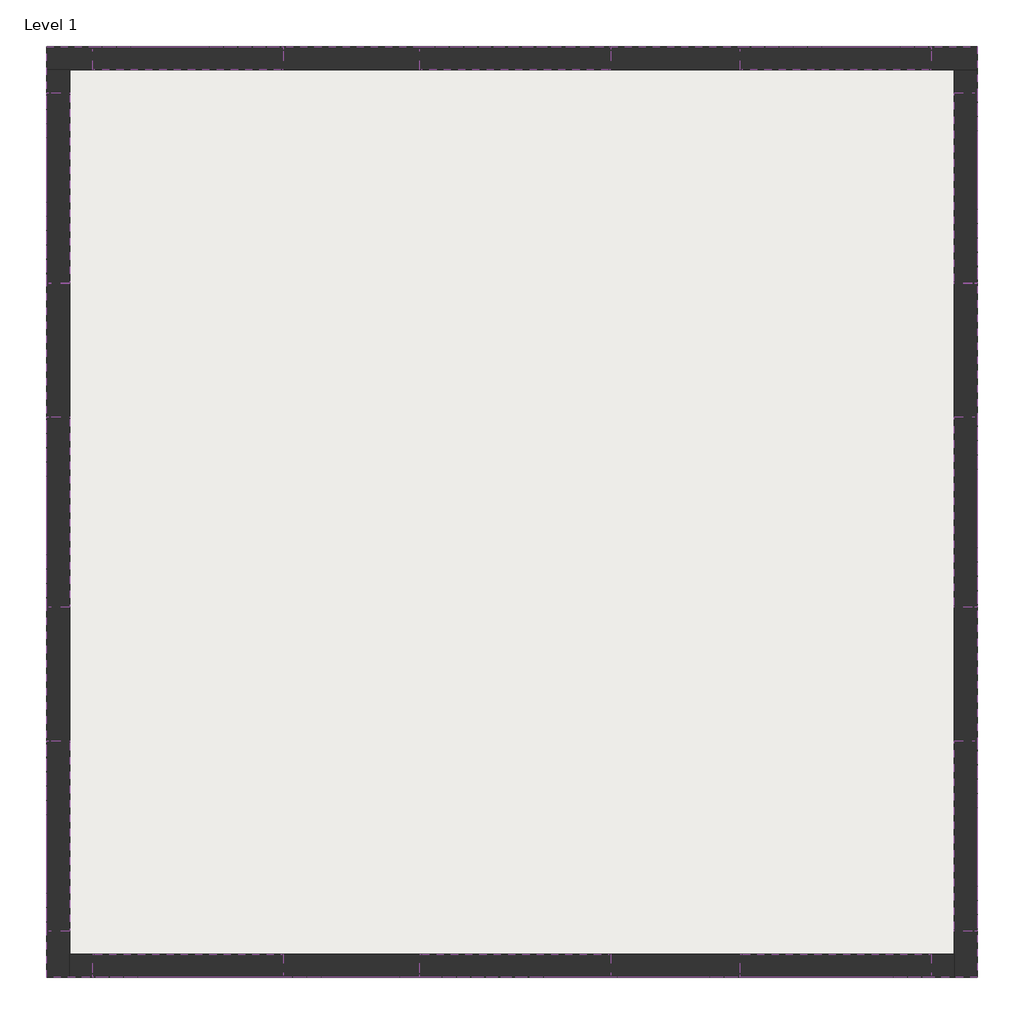
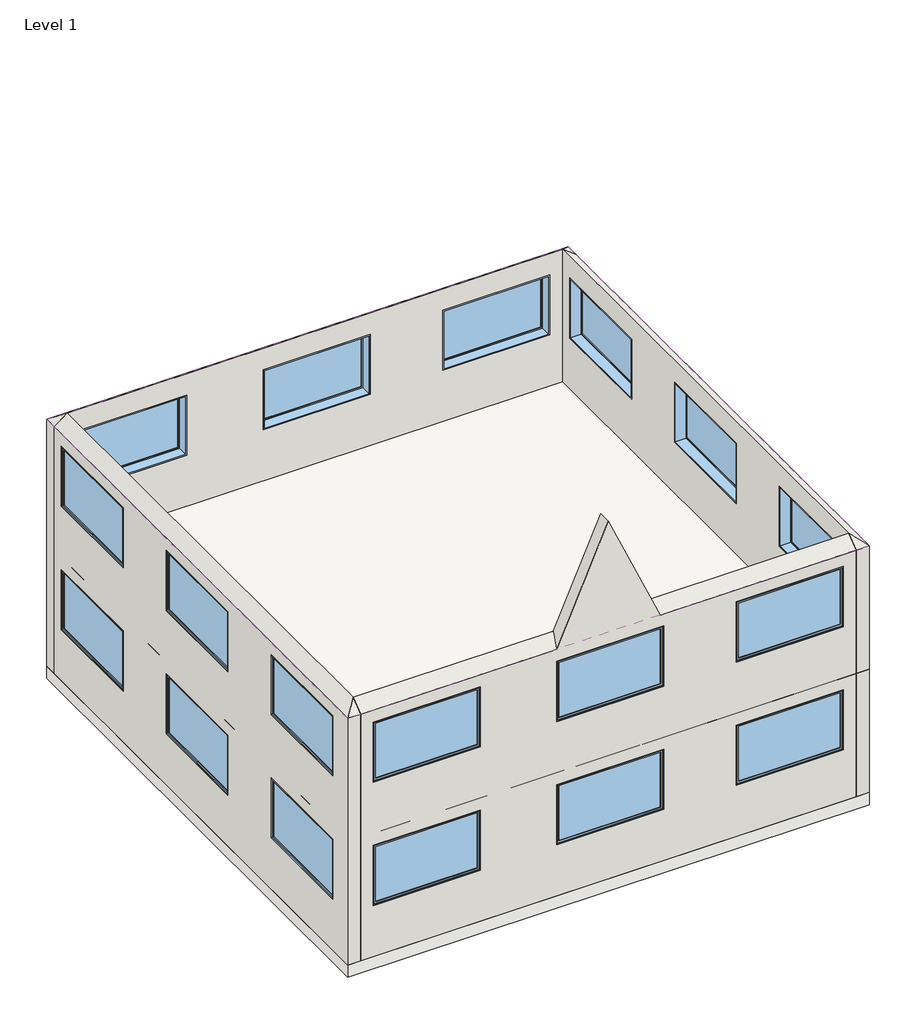
# One storey: 24 windows, 4 walls, 2 slabs, 1 roof.
"""IFC4 building model written with IfcOpenShell, lengths in millimetres."""

import ifcopenshell
import ifcopenshell.guid

model = None  # the IFC model being written
_history = None  # IfcOwnerHistory: only IFC2X3 demands one
_inside = {}  # id of a spatial element -> (the spatial element, [elements in it])
_under = {}  # id of a project, library or spatial element -> (it, [spatial elements below it])
_declared = {}  # id of a project -> (the project, [libraries it declares])
_typed = {}  # id of a type object -> (the type object, [elements of that type])
_made_of = {}  # id of a material, layer set ... -> (it, [elements and type objects made of it])


def new_model(schema):
    """Start an empty IFC model of exactly this schema.

    Asked for "IFC4X3", IfcOpenShell would pick the latest addendum, in which some entities
    have other attributes; the version numbers below select the first issue.
    IFC2X3 requires an IfcOwnerHistory on every rooted entity: one is made here for all.
    """
    global model, _history
    if schema == "IFC4X3":
        model = ifcopenshell.file(schema_version=(4, 3, 0, 0))
    else:
        model = ifcopenshell.file(schema=schema)
    _inside.clear()
    _under.clear()
    _declared.clear()
    _typed.clear()
    _made_of.clear()
    _history = None
    if model.schema == "IFC2X3":
        org = make("IfcOrganization", Name="unknown")
        user = make(
            "IfcPersonAndOrganization",
            ThePerson=make("IfcPerson", FamilyName="unknown"),
            TheOrganization=org,
        )
        app = make(
            "IfcApplication",
            ApplicationDeveloper=org,
            Version="unknown",
            ApplicationFullName="unknown",
            ApplicationIdentifier="unknown",
        )
        _history = make(
            "IfcOwnerHistory",
            OwningUser=user,
            OwningApplication=app,
            ChangeAction="ADDED",
            CreationDate=0,
        )
    return model


def make(cls, **values):
    """One entity of the class cls with the attributes given. An attribute that is None is left unset."""
    return model.create_entity(
        cls, **{name: value for name, value in values.items() if value is not None}
    )


def rooted(cls, **values):
    """An entity with a GlobalId (a new one), such as an element, a storey or a relation."""
    return make(cls, GlobalId=ifcopenshell.guid.new(), OwnerHistory=_history, **values)


def si_unit(unit_type, name, prefix=None):
    """IfcSIUnit, for example si_unit("LENGTHUNIT", "METRE", prefix="MILLI")."""
    return make("IfcSIUnit", UnitType=unit_type, Prefix=prefix, Name=name)


def assignment(units):
    """IfcUnitAssignment: the units of a project."""
    return None if units is None else make("IfcUnitAssignment", Units=units)


def point(xyz):
    """IfcCartesianPoint."""
    return None if xyz is None else make("IfcCartesianPoint", Coordinates=xyz)


def direction(xyz):
    """IfcDirection."""
    return None if xyz is None else make("IfcDirection", DirectionRatios=xyz)


def frame(location, z_axis=None, x_axis=None):
    """IfcAxis2Placement3D, a coordinate frame: its origin and axes. An axis left out is left unset."""
    return make(
        "IfcAxis2Placement3D",
        Location=point(location),
        Axis=direction(z_axis),
        RefDirection=direction(x_axis),
    )


def origin():
    """The frame at (0, 0, 0) with its axes left unset."""
    return frame((0.0, 0.0, 0.0))


def place(relative_to, where):
    """IfcLocalPlacement: puts the frame where relative to a parent placement (None: the world)."""
    return make(
        "IfcLocalPlacement", PlacementRelTo=relative_to, RelativePlacement=where
    )


def context(
    kind, dimensions, precision=None, world=None, true_north=None, identifier=None
):
    """IfcGeometricRepresentationContext, for example the 3D "Model" context."""
    return make(
        "IfcGeometricRepresentationContext",
        ContextIdentifier=identifier,
        ContextType=kind,
        CoordinateSpaceDimension=dimensions,
        Precision=precision,
        WorldCoordinateSystem=world,
        TrueNorth=true_north,
    )


def project(units=None, contexts=None):
    """IfcProject with its units and contexts."""
    return rooted(
        "IfcProject",
        Name="project",
        RepresentationContexts=contexts,
        UnitsInContext=assignment(units),
    )


def spatial(cls, under=None, at=None, **own):
    """A site, building, storey or space (cls), placed at a placement, below another one or the project."""
    s = rooted(cls, ObjectPlacement=at, **own)
    if under is not None:
        _under.setdefault(under.id(), (under, []))[1].append(s)
    return s


def polyline(points):
    """IfcPolyline through the points."""
    return make("IfcPolyline", Points=[point(p) for p in points])


def outline(outer, holes=None, kind="AREA"):
    """IfcArbitraryClosedProfileDef: a profile drawn as a closed curve; with holes, ...WithVoids."""
    if holes is None:
        return make("IfcArbitraryClosedProfileDef", ProfileType=kind, OuterCurve=outer)
    return make(
        "IfcArbitraryProfileDefWithVoids",
        ProfileType=kind,
        OuterCurve=outer,
        InnerCurves=holes,
    )


def extrude(swept, where, along, depth):
    """IfcExtrudedAreaSolid: the profile swept, set in the frame where, extruded along a direction by depth."""
    return make(
        "IfcExtrudedAreaSolid",
        SweptArea=swept,
        Position=where,
        ExtrudedDirection=direction(along),
        Depth=depth,
    )


def faces_of(points, faces, orient=None, outer=None):
    """IfcFace entities. A face is a list of loops; a loop is a list of indices into points, from 0.

    orient and outer hold one flag for each loop. By default every Orientation is true, the
    first loop of a face is its IfcFaceOuterBound and the others are IfcFaceBound.
    """
    made = []
    for i, loops in enumerate(faces):
        bounds = []
        for j, loop in enumerate(loops):
            is_outer = j == 0 if outer is None else outer[i][j]
            bounds.append(
                make(
                    "IfcFaceOuterBound" if is_outer else "IfcFaceBound",
                    Bound=make("IfcPolyLoop", Polygon=[points[k] for k in loop]),
                    Orientation=True if orient is None else orient[i][j],
                )
            )
        made.append(make("IfcFace", Bounds=bounds))
    return made


def faceted_brep(points, faces, orient=None, outer=None, voids=None):
    """IfcFacetedBrep: a solid bounded by flat faces; with voids (closed shells), ...WithVoids."""
    shared = [point(p) for p in points]
    hull = make("IfcClosedShell", CfsFaces=faces_of(shared, faces, orient, outer))
    if voids is None:
        return make("IfcFacetedBrep", Outer=hull)
    return make(
        "IfcFacetedBrepWithVoids",
        Outer=hull,
        Voids=[
            make(cls, CfsFaces=faces_of(shared, fs, o, b)) for cls, fs, o, b in voids
        ],
    )


def shape(context_of_items, identifier, shape_type, items):
    """IfcShapeRepresentation: the items that make up one representation, for example the "Body"."""
    return make(
        "IfcShapeRepresentation",
        ContextOfItems=context_of_items,
        RepresentationIdentifier=identifier,
        RepresentationType=shape_type,
        Items=items,
    )


def source(mapping_origin, context_of_items, identifier, shape_type, items):
    """IfcRepresentationMap: a shape defined once, which mapped items show again and again."""
    return make(
        "IfcRepresentationMap",
        MappingOrigin=mapping_origin,
        MappedRepresentation=shape(context_of_items, identifier, shape_type, items),
    )


def transform(
    local_origin,
    x_axis=None,
    y_axis=None,
    z_axis=None,
    scale=None,
    scale2=None,
    scale3=None,
    uniform=True,
):
    """IfcCartesianTransformationOperator3D, or its non-uniform kind. x_axis, y_axis, z_axis: its Axis1, 2, 3."""
    if uniform:
        return make(
            "IfcCartesianTransformationOperator3D",
            Axis1=direction(x_axis),
            Axis2=direction(y_axis),
            LocalOrigin=point(local_origin),
            Scale=scale,
            Axis3=direction(z_axis),
        )
    return make(
        "IfcCartesianTransformationOperator3DnonUniform",
        Axis1=direction(x_axis),
        Axis2=direction(y_axis),
        LocalOrigin=point(local_origin),
        Scale=scale,
        Axis3=direction(z_axis),
        Scale2=scale2,
        Scale3=scale3,
    )


def mapped(mapping_source, mapping_target):
    """IfcMappedItem: shows the shape of a source again, moved by a transform."""
    return make(
        "IfcMappedItem", MappingSource=mapping_source, MappingTarget=mapping_target
    )


def made_of(thing, what):
    """Note that an element or type object is made of a material, layer set ...; save() writes the relation."""
    if what is not None:
        _made_of.setdefault(what.id(), (what, []))[1].append(thing)
    return thing


def element(
    cls,
    number,
    at=None,
    inside=None,
    cuts=None,
    type_object=None,
    material=None,
    context=None,
    identifier="Body",
    shape_type=None,
    held_by="IfcProductDefinitionShape",
    body=None,
    shapes=None,
    **own,
):
    """One element of the class cls, such as IfcWall. Its Tag is "e" and its number.

    at: its placement. inside: the storey or other place that contains it. cuts: it is an
    opening in that element (IfcRelVoidsElement). A single representation is given by context,
    identifier, shape_type and body (its items); several are given by shapes. held_by: the class
    of the entity that holds the representations. save() writes the other relations.
    """
    e = rooted(cls, Tag="e%d" % number, ObjectPlacement=at, **own)
    if body is not None:
        shapes = [shape(context, identifier, shape_type, body)]
    if shapes is not None:
        e.Representation = make(held_by, Representations=shapes)
    if inside is not None:
        _inside.setdefault(inside.id(), (inside, []))[1].append(e)
    if cuts is not None:
        rooted(
            "IfcRelVoidsElement", RelatingBuildingElement=cuts, RelatedOpeningElement=e
        )
    if type_object is not None:
        _typed.setdefault(type_object.id(), (type_object, []))[1].append(e)
    return made_of(e, material)


def aggregate(whole, parts):
    """IfcRelAggregates: a whole, such as a stair, and the parts it consists of."""
    return rooted("IfcRelAggregates", RelatingObject=whole, RelatedObjects=parts)


def save(model, path):
    """Write the relations noted so far, then the file.

    IfcRelAggregates (storeys below a building ...), IfcRelContainedInSpatialStructure (elements
    in a storey), IfcRelDefinesByType, IfcRelAssociatesMaterial and IfcRelDeclares: one each for
    every whole, place, type object, material and project.
    """
    for whole, parts in _under.values():
        aggregate(whole, parts)
    for where, things in _inside.values():
        rooted(
            "IfcRelContainedInSpatialStructure",
            RelatedElements=things,
            RelatingStructure=where,
        )
    for kind, things in _typed.values():
        rooted("IfcRelDefinesByType", RelatedObjects=things, RelatingType=kind)
    for what, things in _made_of.values():
        rooted("IfcRelAssociatesMaterial", RelatedObjects=things, RelatingMaterial=what)
    for by, libraries in _declared.values():
        rooted("IfcRelDeclares", RelatingContext=by, RelatedDefinitions=libraries)
    model.write(path)


def m_fixed_2500_x_1486mm_baf7df51(model_context):
    return source(origin(), model_context, "Body", "SweptSolid", [
        extrude(outline(polyline([(-1187.0, 130.4), (1187.0, 130.4), (1187.0, 118.4), (-1187.0, 118.4), (-1187.0, 130.4)])), frame((0.0, 0.0, 978.0), z_axis=(0.0, 0.0, 1.0), x_axis=(1.0, 0.0, 0.0)), (0.0, 0.0, 1.0), 1360.5),
        extrude(outline(polyline([(2382.5, -1231.0), (934.0, -1231.0), (934.0, 1231.0), (2382.5, 1231.0), (2382.5, -1231.0)]), holes=[polyline([(2338.5, -1187.0), (2338.5, 1187.0), (978.0, 1187.0), (978.0, -1187.0), (2338.5, -1187.0)])]), frame((0.0, 102.4, 0.0), z_axis=(0.0, 1.0, 0.0), x_axis=(0.0, 0.0, 1.0)), (0.0, 0.0, 1.0), 44.0),
        extrude(outline(polyline([(2401.5, -1250.0), (915.0, -1250.0), (915.0, 1250.0), (2401.5, 1250.0), (2401.5, -1250.0)]), holes=[polyline([(2382.5, -1231.0), (2382.5, 1231.0), (934.0, 1231.0), (934.0, -1231.0), (2382.5, -1231.0)])]), frame((0.0, 102.4, 0.0), z_axis=(0.0, 1.0, 0.0), x_axis=(0.0, 0.0, 1.0)), (0.0, 0.0, 1.0), 63.0),
        extrude(outline(polyline([(2401.5, -1250.0), (915.0, -1250.0), (915.0, 1250.0), (2401.5, 1250.0), (2401.5, -1250.0)]), holes=[polyline([(2369.5, -1218.0), (2369.5, 1218.0), (947.0, 1218.0), (947.0, -1218.0), (2369.5, -1218.0)])]), frame((0.0, -139.4, 0.0), z_axis=(0.0, 1.0, 0.0), x_axis=(0.0, 0.0, 1.0)), (0.0, 0.0, 1.0), 241.8),
    ])


def m_fixed_2500_x_1486mm_49bc14c1(model_context):
    return source(origin(), model_context, "Body", "SweptSolid", [
        extrude(outline(polyline([(-1187.0, -130.4), (-1187.0, -118.4), (1187.0, -118.4), (1187.0, -130.4), (-1187.0, -130.4)])), frame((0.0, 0.0, 978.0), z_axis=(0.0, 0.0, 1.0), x_axis=(1.0, 0.0, 0.0)), (0.0, 0.0, 1.0), 1360.5),
        extrude(outline(polyline([(2382.5, -1231.0), (934.0, -1231.0), (934.0, 1231.0), (2382.5, 1231.0), (2382.5, -1231.0)]), holes=[polyline([(2338.5, -1187.0), (2338.5, 1187.0), (978.0, 1187.0), (978.0, -1187.0), (2338.5, -1187.0)])]), frame((0.0, -146.4, 0.0), z_axis=(0.0, 1.0, 0.0), x_axis=(0.0, 0.0, 1.0)), (0.0, 0.0, 1.0), 44.0),
        extrude(outline(polyline([(2401.5, -1250.0), (915.0, -1250.0), (915.0, 1250.0), (2401.5, 1250.0), (2401.5, -1250.0)]), holes=[polyline([(2382.5, -1231.0), (2382.5, 1231.0), (934.0, 1231.0), (934.0, -1231.0), (2382.5, -1231.0)])]), frame((0.0, -165.4, 0.0), z_axis=(0.0, 1.0, 0.0), x_axis=(0.0, 0.0, 1.0)), (0.0, 0.0, 1.0), 63.0),
        extrude(outline(polyline([(2401.5, -1250.0), (915.0, -1250.0), (915.0, 1250.0), (2401.5, 1250.0), (2401.5, -1250.0)]), holes=[polyline([(2369.5, -1218.0), (2369.5, 1218.0), (947.0, 1218.0), (947.0, -1218.0), (2369.5, -1218.0)])]), frame((0.0, -102.4, 0.0), z_axis=(0.0, 1.0, 0.0), x_axis=(0.0, 0.0, 1.0)), (0.0, 0.0, 1.0), 241.8),
    ])


model = new_model("IFC4")

# Units and contexts
model_context = context("Model", 3, world=origin())
ifc_project = project(units=[si_unit("LENGTHUNIT", "METRE", prefix="MILLI")], contexts=[model_context])

# Site, building, storey
site = spatial("IfcSite", under=ifc_project)
building = spatial("IfcBuilding", under=site)
storey = spatial("IfcBuildingStorey", under=building, Name="Level 1", Elevation=0.0)

# Roof
placement = place(None, origin())
element("IfcRoof", 1, ObjectType="Generic Roof - 300mm", at=placement, inside=storey, context=model_context, shape_type="Brep", body=[
    faceted_brep([(21465.644102, 9062.7173115, 6096.0), (15369.644102, 2966.7173115, 10668.0170156), (9273.644102, 9062.7173115, 6096.0), (9273.644102, -3129.2826885, 6096.0), (14160.6176554, -3129.2826885, 6096.0), (13998.044102, -3129.2826885, 6096.0), (21465.644102, -3129.2826885, 6096.0), (16741.244102, -3129.2826885, 6096.0), (16578.6705485, -3129.2826885, 6096.0), (15369.644102, 528.4582497, 8839.3159134), (15369.644102, -3129.2826885, 8839.3159134), (21465.644102, 9062.7173115, 6471.0005024), (9273.644102, 9062.7173115, 6471.0005024), (15369.644102, 2966.7173115, 11043.0175181), (9273.644102, -3129.2826885, 6471.0005024), (13998.044102, -3129.2826885, 6471.0005024), (15369.644102, 1020.3018679, 9583.2005024), (16741.244102, -3129.2826885, 6471.0005024), (21465.644102, -3129.2826885, 6471.0005024), (15369.644102, -3129.2826885, 9583.2005024)], [[[0, 1, 2]], [[2, 1, 3]], [[4, 5, 3, 1, 6, 7, 8, 9]], [[6, 1, 0]], [[4, 9, 10]], [[8, 10, 9]], [[11, 12, 13]], [[12, 14, 13]], [[15, 16, 17, 18, 13, 14]], [[18, 11, 13]], [[15, 19, 16]], [[17, 16, 19]], [[6, 18, 17, 7]], [[0, 11, 18, 6]], [[2, 12, 11, 0]], [[3, 14, 12, 2]], [[5, 15, 14, 3]], [[17, 19, 15, 5, 4, 10, 8, 7]]]),
])

# Slabs
element("IfcSlab", 2, ObjectType="Generic Floor - 304.8mm", at=placement, inside=storey, context=model_context, shape_type="Brep", body=[
    faceted_brep([(21465.644102, 9062.7173115, -304.8), (21465.644102, -3129.2826885, -304.8), (9273.644102, -3129.2826885, -304.8), (9273.644102, 9062.7173115, -304.8), (21465.644102, 9062.7173115, 0.0), (9273.644102, 9062.7173115, 0.0), (9273.644102, -3129.2826885, 0.0), (9578.444102, -3129.2826885, 0.0), (21160.844102, -3129.2826885, 0.0), (21465.644102, -3129.2826885, 0.0), (21465.644102, 8757.9173115, 0.0)], [[[0, 1, 2, 3]], [[4, 5, 6, 7, 8, 9, 10]], [[1, 0, 4, 10, 9]], [[2, 1, 9, 8, 7, 6]], [[3, 2, 6, 5]], [[0, 3, 5, 4]]]),
])
element("IfcSlab", 3, ObjectType="Generic Floor - 304.8mm", at=placement, inside=storey, context=model_context, shape_type="SweptSolid", body=[
    extrude(outline(polyline([(21465.644102, 9062.7173115), (21465.644102, -3129.2826885), (9273.644102, -3129.2826885), (9273.644102, 9062.7173115), (21465.644102, 9062.7173115)])), frame((0.0, 0.0, 2743.2), z_axis=(0.0, 0.0, 1.0), x_axis=(1.0, 0.0, 0.0)), (0.0, 0.0, 1.0), 304.8),
])

# Walls
element("IfcWall", 4, ObjectType="Generic - 304.8mm", at=placement, inside=storey, context=model_context, shape_type="Brep", body=[
    faceted_brep([(9273.644102, 8757.9173115, 0.0), (9578.444102, 8757.9173115, 0.0), (21160.844102, 8757.9173115, 0.0), (21465.644102, 8757.9173115, 0.0), (21465.644102, 8757.9173115, 6096.0), (21160.844102, 8757.9173115, 6324.6008508), (9578.444102, 8757.9173115, 6324.6008508), (9273.644102, 8757.9173115, 6096.0), (14163.244102, 8757.9173115, 4309.5), (14163.244102, 8757.9173115, 5796.0), (16663.244102, 8757.9173115, 5796.0), (16663.244102, 8757.9173115, 4309.5), (9876.044102, 8757.9173115, 4309.5), (9876.044102, 8757.9173115, 5796.0), (12376.044102, 8757.9173115, 5796.0), (12376.044102, 8757.9173115, 4309.5), (18363.244102, 8757.9173115, 4309.5), (18363.244102, 8757.9173115, 5796.0), (20863.244102, 8757.9173115, 5796.0), (20863.244102, 8757.9173115, 4309.5), (18363.244102, 8757.9173115, 1261.5), (18363.244102, 8757.9173115, 2748.0), (20863.244102, 8757.9173115, 2748.0), (20863.244102, 8757.9173115, 1261.5), (9876.044102, 8757.9173115, 1261.5), (9876.044102, 8757.9173115, 2748.0), (12376.044102, 8757.9173115, 2748.0), (12376.044102, 8757.9173115, 1261.5), (14163.244102, 8757.9173115, 1261.5), (14163.244102, 8757.9173115, 2748.0), (16663.244102, 8757.9173115, 2748.0), (16663.244102, 8757.9173115, 1261.5), (9273.644102, 9062.7173115, 0.0), (9273.644102, 9062.7173115, 6096.0), (21465.644102, 9062.7173115, 6096.0), (21465.644102, 9062.7173115, 0.0), (14163.244102, 9062.7173115, 4309.5), (16663.244102, 9062.7173115, 4309.5), (16663.244102, 9062.7173115, 5796.0), (14163.244102, 9062.7173115, 5796.0), (9876.044102, 9062.7173115, 4309.5), (12376.044102, 9062.7173115, 4309.5), (12376.044102, 9062.7173115, 5796.0), (9876.044102, 9062.7173115, 5796.0), (18363.244102, 9062.7173115, 4309.5), (20863.244102, 9062.7173115, 4309.5), (20863.244102, 9062.7173115, 5796.0), (18363.244102, 9062.7173115, 5796.0), (18363.244102, 9062.7173115, 1261.5), (20863.244102, 9062.7173115, 1261.5), (20863.244102, 9062.7173115, 2748.0), (18363.244102, 9062.7173115, 2748.0), (9876.044102, 9062.7173115, 1261.5), (12376.044102, 9062.7173115, 1261.5), (12376.044102, 9062.7173115, 2748.0), (9876.044102, 9062.7173115, 2748.0), (14163.244102, 9062.7173115, 1261.5), (16663.244102, 9062.7173115, 1261.5), (16663.244102, 9062.7173115, 2748.0), (14163.244102, 9062.7173115, 2748.0)], [[[0, 1, 2, 3, 4, 5, 6, 7], [8, 9, 10, 11], [12, 13, 14, 15], [16, 17, 18, 19], [20, 21, 22, 23], [24, 25, 26, 27], [28, 29, 30, 31]], [[32, 33, 34, 35], [36, 37, 38, 39], [40, 41, 42, 43], [44, 45, 46, 47], [48, 49, 50, 51], [52, 53, 54, 55], [56, 57, 58, 59]], [[3, 2, 1, 0, 32, 35]], [[4, 3, 35, 34]], [[0, 7, 33, 32]], [[9, 8, 36, 39]], [[10, 9, 39, 38]], [[11, 10, 38, 37]], [[8, 11, 37, 36]], [[13, 12, 40, 43]], [[14, 13, 43, 42]], [[15, 14, 42, 41]], [[12, 15, 41, 40]], [[17, 16, 44, 47]], [[18, 17, 47, 46]], [[19, 18, 46, 45]], [[16, 19, 45, 44]], [[21, 20, 48, 51]], [[22, 21, 51, 50]], [[23, 22, 50, 49]], [[20, 23, 49, 48]], [[25, 24, 52, 55]], [[26, 25, 55, 54]], [[27, 26, 54, 53]], [[24, 27, 53, 52]], [[29, 28, 56, 59]], [[30, 29, 59, 58]], [[31, 30, 58, 57]], [[28, 31, 57, 56]], [[7, 6, 33]], [[6, 5, 34, 33]], [[5, 4, 34]]]),
])
element("IfcWall", 5, ObjectType="Generic - 304.8mm", at=placement, inside=storey, context=model_context, shape_type="Brep", body=[
    faceted_brep([(21160.844102, 8757.9173115, 0.0), (21160.844102, -2824.4826885, 0.0), (21160.844102, -3129.2826885, 0.0), (21160.844102, -3129.2826885, 6096.0), (21160.844102, -2824.4826885, 6324.6008508), (21160.844102, 8757.9173115, 6324.6008508), (21160.844102, -26.8826885, 4309.5), (21160.844102, -26.8826885, 5796.0), (21160.844102, -2526.8826885, 5796.0), (21160.844102, -2526.8826885, 4309.5), (21160.844102, 8460.3173115, 4309.5), (21160.844102, 8460.3173115, 5796.0), (21160.844102, 5960.3173115, 5796.0), (21160.844102, 5960.3173115, 4309.5), (21160.844102, 4216.7173115, 4309.5), (21160.844102, 4216.7173115, 5796.0), (21160.844102, 1716.7173115, 5796.0), (21160.844102, 1716.7173115, 4309.5), (21160.844102, 4216.7173115, 1261.5), (21160.844102, 4216.7173115, 2748.0), (21160.844102, 1716.7173115, 2748.0), (21160.844102, 1716.7173115, 1261.5), (21160.844102, 8460.3173115, 1261.5), (21160.844102, 8460.3173115, 2748.0), (21160.844102, 5960.3173115, 2748.0), (21160.844102, 5960.3173115, 1261.5), (21160.844102, -26.8826885, 1261.5), (21160.844102, -26.8826885, 2748.0), (21160.844102, -2526.8826885, 2748.0), (21160.844102, -2526.8826885, 1261.5), (21465.644102, 8757.9173115, 0.0), (21465.644102, 8757.9173115, 6096.0), (21465.644102, -3129.2826885, 6096.0), (21465.644102, -3129.2826885, 0.0), (21465.644102, -26.8826885, 4309.5), (21465.644102, -2526.8826885, 4309.5), (21465.644102, -2526.8826885, 5796.0), (21465.644102, -26.8826885, 5796.0), (21465.644102, 8460.3173115, 4309.5), (21465.644102, 5960.3173115, 4309.5), (21465.644102, 5960.3173115, 5796.0), (21465.644102, 8460.3173115, 5796.0), (21465.644102, 4216.7173115, 4309.5), (21465.644102, 1716.7173115, 4309.5), (21465.644102, 1716.7173115, 5796.0), (21465.644102, 4216.7173115, 5796.0), (21465.644102, 4216.7173115, 1261.5), (21465.644102, 1716.7173115, 1261.5), (21465.644102, 1716.7173115, 2748.0), (21465.644102, 4216.7173115, 2748.0), (21465.644102, 8460.3173115, 1261.5), (21465.644102, 5960.3173115, 1261.5), (21465.644102, 5960.3173115, 2748.0), (21465.644102, 8460.3173115, 2748.0), (21465.644102, -26.8826885, 1261.5), (21465.644102, -2526.8826885, 1261.5), (21465.644102, -2526.8826885, 2748.0), (21465.644102, -26.8826885, 2748.0)], [[[0, 1, 2, 3, 4, 5], [6, 7, 8, 9], [10, 11, 12, 13], [14, 15, 16, 17], [18, 19, 20, 21], [22, 23, 24, 25], [26, 27, 28, 29]], [[30, 31, 32, 33], [34, 35, 36, 37], [38, 39, 40, 41], [42, 43, 44, 45], [46, 47, 48, 49], [50, 51, 52, 53], [54, 55, 56, 57]], [[2, 1, 0, 30, 33]], [[0, 5, 31, 30]], [[3, 2, 33, 32]], [[7, 6, 34, 37]], [[8, 7, 37, 36]], [[9, 8, 36, 35]], [[6, 9, 35, 34]], [[11, 10, 38, 41]], [[12, 11, 41, 40]], [[13, 12, 40, 39]], [[10, 13, 39, 38]], [[15, 14, 42, 45]], [[16, 15, 45, 44]], [[17, 16, 44, 43]], [[14, 17, 43, 42]], [[19, 18, 46, 49]], [[20, 19, 49, 48]], [[21, 20, 48, 47]], [[18, 21, 47, 46]], [[23, 22, 50, 53]], [[24, 23, 53, 52]], [[25, 24, 52, 51]], [[22, 25, 51, 50]], [[27, 26, 54, 57]], [[28, 27, 57, 56]], [[29, 28, 56, 55]], [[26, 29, 55, 54]], [[5, 4, 32, 31]], [[4, 3, 32]]]),
])
element("IfcWall", 6, ObjectType="Generic - 304.8mm", at=placement, inside=storey, context=model_context, shape_type="Brep", body=[
    faceted_brep([(9578.444102, -3129.2826885, 0.0), (9578.444102, -2824.4826885, 0.0), (9578.444102, 8757.9173115, 0.0), (9578.444102, 8757.9173115, 6324.6008508), (9578.444102, -2824.4826885, 6324.6008508), (9578.444102, -3129.2826885, 6096.0), (9578.444102, 1716.7173115, 4309.5), (9578.444102, 1716.7173115, 5796.0), (9578.444102, 4216.7173115, 5796.0), (9578.444102, 4216.7173115, 4309.5), (9578.444102, 5960.3173115, 4309.5), (9578.444102, 5960.3173115, 5796.0), (9578.444102, 8460.3173115, 5796.0), (9578.444102, 8460.3173115, 4309.5), (9578.444102, -2526.8826885, 4309.5), (9578.444102, -2526.8826885, 5796.0), (9578.444102, -26.8826885, 5796.0), (9578.444102, -26.8826885, 4309.5), (9578.444102, -2526.8826885, 1261.5), (9578.444102, -2526.8826885, 2748.0), (9578.444102, -26.8826885, 2748.0), (9578.444102, -26.8826885, 1261.5), (9578.444102, 5960.3173115, 1261.5), (9578.444102, 5960.3173115, 2748.0), (9578.444102, 8460.3173115, 2748.0), (9578.444102, 8460.3173115, 1261.5), (9578.444102, 1716.7173115, 1261.5), (9578.444102, 1716.7173115, 2748.0), (9578.444102, 4216.7173115, 2748.0), (9578.444102, 4216.7173115, 1261.5), (9273.644102, -3129.2826885, 0.0), (9273.644102, -3129.2826885, 6096.0), (9273.644102, 8757.9173115, 6096.0), (9273.644102, 8757.9173115, 0.0), (9273.644102, 1716.7173115, 4309.5), (9273.644102, 4216.7173115, 4309.5), (9273.644102, 4216.7173115, 5796.0), (9273.644102, 1716.7173115, 5796.0), (9273.644102, 5960.3173115, 4309.5), (9273.644102, 8460.3173115, 4309.5), (9273.644102, 8460.3173115, 5796.0), (9273.644102, 5960.3173115, 5796.0), (9273.644102, -2526.8826885, 4309.5), (9273.644102, -26.8826885, 4309.5), (9273.644102, -26.8826885, 5796.0), (9273.644102, -2526.8826885, 5796.0), (9273.644102, -2526.8826885, 1261.5), (9273.644102, -26.8826885, 1261.5), (9273.644102, -26.8826885, 2748.0), (9273.644102, -2526.8826885, 2748.0), (9273.644102, 5960.3173115, 1261.5), (9273.644102, 8460.3173115, 1261.5), (9273.644102, 8460.3173115, 2748.0), (9273.644102, 5960.3173115, 2748.0), (9273.644102, 1716.7173115, 1261.5), (9273.644102, 4216.7173115, 1261.5), (9273.644102, 4216.7173115, 2748.0), (9273.644102, 1716.7173115, 2748.0)], [[[0, 1, 2, 3, 4, 5], [6, 7, 8, 9], [10, 11, 12, 13], [14, 15, 16, 17], [18, 19, 20, 21], [22, 23, 24, 25], [26, 27, 28, 29]], [[30, 31, 32, 33], [34, 35, 36, 37], [38, 39, 40, 41], [42, 43, 44, 45], [46, 47, 48, 49], [50, 51, 52, 53], [54, 55, 56, 57]], [[2, 1, 0, 30, 33]], [[3, 2, 33, 32]], [[0, 5, 31, 30]], [[7, 6, 34, 37]], [[8, 7, 37, 36]], [[9, 8, 36, 35]], [[6, 9, 35, 34]], [[11, 10, 38, 41]], [[12, 11, 41, 40]], [[13, 12, 40, 39]], [[10, 13, 39, 38]], [[15, 14, 42, 45]], [[16, 15, 45, 44]], [[17, 16, 44, 43]], [[14, 17, 43, 42]], [[19, 18, 46, 49]], [[20, 19, 49, 48]], [[21, 20, 48, 47]], [[18, 21, 47, 46]], [[23, 22, 50, 53]], [[24, 23, 53, 52]], [[25, 24, 52, 51]], [[22, 25, 51, 50]], [[27, 26, 54, 57]], [[28, 27, 57, 56]], [[29, 28, 56, 55]], [[26, 29, 55, 54]], [[5, 4, 31]], [[4, 3, 32, 31]]]),
])
element("IfcWall", 7, ObjectType="Generic - 304.8mm", at=placement, inside=storey, context=model_context, shape_type="Brep", body=[
    faceted_brep([(9578.444102, -3129.2826885, 0.0), (21160.844102, -3129.2826885, 0.0), (21160.844102, -3129.2826885, 6096.0), (16741.244102, -3129.2826885, 6096.0), (16578.6705485, -3129.2826885, 6096.0), (15369.644102, -3129.2826885, 8839.3159134), (14160.6176554, -3129.2826885, 6096.0), (13998.044102, -3129.2826885, 6096.0), (9578.444102, -3129.2826885, 6096.0), (14163.244102, -3129.2826885, 4309.5), (14163.244102, -3129.2826885, 5796.0), (16663.244102, -3129.2826885, 5796.0), (16663.244102, -3129.2826885, 4309.5), (9876.044102, -3129.2826885, 4309.5), (9876.044102, -3129.2826885, 5796.0), (12376.044102, -3129.2826885, 5796.0), (12376.044102, -3129.2826885, 4309.5), (18363.244102, -3129.2826885, 4309.5), (18363.244102, -3129.2826885, 5796.0), (20863.244102, -3129.2826885, 5796.0), (20863.244102, -3129.2826885, 4309.5), (18363.244102, -3129.2826885, 1261.5), (18363.244102, -3129.2826885, 2748.0), (20863.244102, -3129.2826885, 2748.0), (20863.244102, -3129.2826885, 1261.5), (9876.044102, -3129.2826885, 1261.5), (9876.044102, -3129.2826885, 2748.0), (12376.044102, -3129.2826885, 2748.0), (12376.044102, -3129.2826885, 1261.5), (14163.244102, -3129.2826885, 1261.5), (14163.244102, -3129.2826885, 2748.0), (16663.244102, -3129.2826885, 2748.0), (16663.244102, -3129.2826885, 1261.5), (9578.444102, -2824.4826885, 0.0), (9578.444102, -2824.4826885, 6324.6008508), (14261.3659772, -2824.4826885, 6324.6008508), (15369.644102, -2824.4826885, 8839.3159134), (16477.9222268, -2824.4826885, 6324.6008508), (21160.844102, -2824.4826885, 6324.6008508), (21160.844102, -2824.4826885, 0.0), (14163.244102, -2824.4826885, 4309.5), (16663.244102, -2824.4826885, 4309.5), (16663.244102, -2824.4826885, 5796.0), (14163.244102, -2824.4826885, 5796.0), (9876.044102, -2824.4826885, 4309.5), (12376.044102, -2824.4826885, 4309.5), (12376.044102, -2824.4826885, 5796.0), (9876.044102, -2824.4826885, 5796.0), (18363.244102, -2824.4826885, 4309.5), (20863.244102, -2824.4826885, 4309.5), (20863.244102, -2824.4826885, 5796.0), (18363.244102, -2824.4826885, 5796.0), (18363.244102, -2824.4826885, 1261.5), (20863.244102, -2824.4826885, 1261.5), (20863.244102, -2824.4826885, 2748.0), (18363.244102, -2824.4826885, 2748.0), (9876.044102, -2824.4826885, 1261.5), (12376.044102, -2824.4826885, 1261.5), (12376.044102, -2824.4826885, 2748.0), (9876.044102, -2824.4826885, 2748.0), (14163.244102, -2824.4826885, 1261.5), (16663.244102, -2824.4826885, 1261.5), (16663.244102, -2824.4826885, 2748.0), (14163.244102, -2824.4826885, 2748.0)], [[[0, 1, 2, 3, 4, 5, 6, 7, 8], [9, 10, 11, 12], [13, 14, 15, 16], [17, 18, 19, 20], [21, 22, 23, 24], [25, 26, 27, 28], [29, 30, 31, 32]], [[33, 34, 35, 36, 37, 38, 39], [40, 41, 42, 43], [44, 45, 46, 47], [48, 49, 50, 51], [52, 53, 54, 55], [56, 57, 58, 59], [60, 61, 62, 63]], [[1, 0, 33, 39]], [[10, 9, 40, 43]], [[11, 10, 43, 42]], [[12, 11, 42, 41]], [[9, 12, 41, 40]], [[14, 13, 44, 47]], [[15, 14, 47, 46]], [[16, 15, 46, 45]], [[13, 16, 45, 44]], [[18, 17, 48, 51]], [[19, 18, 51, 50]], [[20, 19, 50, 49]], [[17, 20, 49, 48]], [[22, 21, 52, 55]], [[23, 22, 55, 54]], [[24, 23, 54, 53]], [[21, 24, 53, 52]], [[26, 25, 56, 59]], [[27, 26, 59, 58]], [[28, 27, 58, 57]], [[25, 28, 57, 56]], [[30, 29, 60, 63]], [[31, 30, 63, 62]], [[32, 31, 62, 61]], [[29, 32, 61, 60]], [[2, 1, 39, 38]], [[0, 8, 34, 33]], [[8, 7, 6, 35, 34]], [[6, 5, 36, 35]], [[5, 4, 37, 36]], [[4, 3, 2, 38, 37]]]),
])

# Windows
m_fixed_2500_x_1486mm_shape = m_fixed_2500_x_1486mm_baf7df51(model_context)
element("IfcWindow", 8, ObjectType="M_Fixed : 2500 x 1486mm", at=placement, inside=storey, context=model_context, shape_type="MappedRepresentation", body=[
    mapped(m_fixed_2500_x_1486mm_shape, transform((15413.244102, 8897.3173115, 3394.5), x_axis=(1.0, 0.0, 0.0), y_axis=(0.0, 1.0, 0.0), z_axis=(0.0, 0.0, 1.0))),
])
element("IfcWindow", 9, ObjectType="M_Fixed : 2500 x 1486mm", at=placement, inside=storey, context=model_context, shape_type="MappedRepresentation", body=[
    mapped(m_fixed_2500_x_1486mm_shape, transform((11126.044102, 8897.3173115, 3394.5), x_axis=(1.0, 0.0, 0.0), y_axis=(0.0, 1.0, 0.0), z_axis=(0.0, 0.0, 1.0))),
])
element("IfcWindow", 10, ObjectType="M_Fixed : 2500 x 1486mm", at=placement, inside=storey, context=model_context, shape_type="MappedRepresentation", body=[
    mapped(m_fixed_2500_x_1486mm_shape, transform((19613.244102, 8897.3173115, 3394.5), x_axis=(1.0, 0.0, 0.0), y_axis=(0.0, 1.0, 0.0), z_axis=(0.0, 0.0, 1.0))),
])
element("IfcWindow", 11, ObjectType="M_Fixed : 2500 x 1486mm", at=placement, inside=storey, context=model_context, shape_type="MappedRepresentation", body=[
    mapped(m_fixed_2500_x_1486mm_shape, transform((15413.244102, 8897.3173115, 346.5), x_axis=(1.0, 0.0, 0.0), y_axis=(0.0, 1.0, 0.0), z_axis=(0.0, 0.0, 1.0))),
])
element("IfcWindow", 12, ObjectType="M_Fixed : 2500 x 1486mm", at=placement, inside=storey, context=model_context, shape_type="MappedRepresentation", body=[
    mapped(m_fixed_2500_x_1486mm_shape, transform((11126.044102, 8897.3173115, 346.5), x_axis=(1.0, 0.0, 0.0), y_axis=(0.0, 1.0, 0.0), z_axis=(0.0, 0.0, 1.0))),
])
element("IfcWindow", 13, ObjectType="M_Fixed : 2500 x 1486mm", at=placement, inside=storey, context=model_context, shape_type="MappedRepresentation", body=[
    mapped(m_fixed_2500_x_1486mm_shape, transform((19613.244102, 8897.3173115, 346.5), x_axis=(1.0, 0.0, 0.0), y_axis=(0.0, 1.0, 0.0), z_axis=(0.0, 0.0, 1.0))),
])
element("IfcWindow", 14, ObjectType="M_Fixed : 2500 x 1486mm", at=placement, inside=storey, context=model_context, shape_type="MappedRepresentation", body=[
    mapped(m_fixed_2500_x_1486mm_shape, transform((21300.244102, -1276.8826885, 3394.5), x_axis=(0.0, -1.0, 0.0), y_axis=(1.0, 0.0, 0.0), z_axis=(0.0, 0.0, 1.0))),
])
element("IfcWindow", 15, ObjectType="M_Fixed : 2500 x 1486mm", at=placement, inside=storey, context=model_context, shape_type="MappedRepresentation", body=[
    mapped(m_fixed_2500_x_1486mm_shape, transform((21300.244102, 7210.3173115, 3394.5), x_axis=(0.0, -1.0, 0.0), y_axis=(1.0, 0.0, 0.0), z_axis=(0.0, 0.0, 1.0))),
])
element("IfcWindow", 16, ObjectType="M_Fixed : 2500 x 1486mm", at=placement, inside=storey, context=model_context, shape_type="MappedRepresentation", body=[
    mapped(m_fixed_2500_x_1486mm_shape, transform((21300.244102, 2966.7173115, 3394.5), x_axis=(0.0, -1.0, 0.0), y_axis=(1.0, 0.0, 0.0), z_axis=(0.0, 0.0, 1.0))),
])
element("IfcWindow", 17, ObjectType="M_Fixed : 2500 x 1486mm", at=placement, inside=storey, context=model_context, shape_type="MappedRepresentation", body=[
    mapped(m_fixed_2500_x_1486mm_shape, transform((21300.244102, -1276.8826885, 346.5), x_axis=(0.0, -1.0, 0.0), y_axis=(1.0, 0.0, 0.0), z_axis=(0.0, 0.0, 1.0))),
])
element("IfcWindow", 18, ObjectType="M_Fixed : 2500 x 1486mm", at=placement, inside=storey, context=model_context, shape_type="MappedRepresentation", body=[
    mapped(m_fixed_2500_x_1486mm_shape, transform((21300.244102, 7210.3173115, 346.5), x_axis=(0.0, -1.0, 0.0), y_axis=(1.0, 0.0, 0.0), z_axis=(0.0, 0.0, 1.0))),
])
element("IfcWindow", 19, ObjectType="M_Fixed : 2500 x 1486mm", at=placement, inside=storey, context=model_context, shape_type="MappedRepresentation", body=[
    mapped(m_fixed_2500_x_1486mm_shape, transform((21300.244102, 2966.7173115, 346.5), x_axis=(0.0, -1.0, 0.0), y_axis=(1.0, 0.0, 0.0), z_axis=(0.0, 0.0, 1.0))),
])
element("IfcWindow", 20, ObjectType="M_Fixed : 2500 x 1486mm", at=placement, inside=storey, context=model_context, shape_type="MappedRepresentation", body=[
    mapped(m_fixed_2500_x_1486mm_shape, transform((9439.044102, 2966.7173115, 3394.5), x_axis=(0.0, 1.0, 0.0), y_axis=(-1.0, 0.0, 0.0), z_axis=(0.0, 0.0, 1.0))),
])
element("IfcWindow", 21, ObjectType="M_Fixed : 2500 x 1486mm", at=placement, inside=storey, context=model_context, shape_type="MappedRepresentation", body=[
    mapped(m_fixed_2500_x_1486mm_shape, transform((9439.044102, 7210.3173115, 3394.5), x_axis=(0.0, 1.0, 0.0), y_axis=(-1.0, 0.0, 0.0), z_axis=(0.0, 0.0, 1.0))),
])
element("IfcWindow", 22, ObjectType="M_Fixed : 2500 x 1486mm", at=placement, inside=storey, context=model_context, shape_type="MappedRepresentation", body=[
    mapped(m_fixed_2500_x_1486mm_shape, transform((9439.044102, -1276.8826885, 3394.5), x_axis=(0.0, 1.0, 0.0), y_axis=(-1.0, 0.0, 0.0), z_axis=(0.0, 0.0, 1.0))),
])
element("IfcWindow", 23, ObjectType="M_Fixed : 2500 x 1486mm", at=placement, inside=storey, context=model_context, shape_type="MappedRepresentation", body=[
    mapped(m_fixed_2500_x_1486mm_shape, transform((9439.044102, 2966.7173115, 346.5), x_axis=(0.0, 1.0, 0.0), y_axis=(-1.0, 0.0, 0.0), z_axis=(0.0, 0.0, 1.0))),
])
element("IfcWindow", 24, ObjectType="M_Fixed : 2500 x 1486mm", at=placement, inside=storey, context=model_context, shape_type="MappedRepresentation", body=[
    mapped(m_fixed_2500_x_1486mm_shape, transform((9439.044102, 7210.3173115, 346.5), x_axis=(0.0, 1.0, 0.0), y_axis=(-1.0, 0.0, 0.0), z_axis=(0.0, 0.0, 1.0))),
])
element("IfcWindow", 25, ObjectType="M_Fixed : 2500 x 1486mm", at=placement, inside=storey, context=model_context, shape_type="MappedRepresentation", body=[
    mapped(m_fixed_2500_x_1486mm_shape, transform((9439.044102, -1276.8826885, 346.5), x_axis=(0.0, 1.0, 0.0), y_axis=(-1.0, 0.0, 0.0), z_axis=(0.0, 0.0, 1.0))),
])
m_fixed_2500_x_1486mm_2_shape = m_fixed_2500_x_1486mm_49bc14c1(model_context)
element("IfcWindow", 26, ObjectType="M_Fixed : 2500 x 1486mm", at=placement, inside=storey, context=model_context, shape_type="MappedRepresentation", body=[
    mapped(m_fixed_2500_x_1486mm_2_shape, transform((15413.244102, -2963.8826885, 3394.5), x_axis=(1.0, 0.0, 0.0), y_axis=(0.0, 1.0, 0.0), z_axis=(0.0, 0.0, 1.0))),
])
element("IfcWindow", 27, ObjectType="M_Fixed : 2500 x 1486mm", at=placement, inside=storey, context=model_context, shape_type="MappedRepresentation", body=[
    mapped(m_fixed_2500_x_1486mm_2_shape, transform((11126.044102, -2963.8826885, 3394.5), x_axis=(1.0, 0.0, 0.0), y_axis=(0.0, 1.0, 0.0), z_axis=(0.0, 0.0, 1.0))),
])
element("IfcWindow", 28, ObjectType="M_Fixed : 2500 x 1486mm", at=placement, inside=storey, context=model_context, shape_type="MappedRepresentation", body=[
    mapped(m_fixed_2500_x_1486mm_2_shape, transform((19613.244102, -2963.8826885, 3394.5), x_axis=(1.0, 0.0, 0.0), y_axis=(0.0, 1.0, 0.0), z_axis=(0.0, 0.0, 1.0))),
])
element("IfcWindow", 29, ObjectType="M_Fixed : 2500 x 1486mm", at=placement, inside=storey, context=model_context, shape_type="MappedRepresentation", body=[
    mapped(m_fixed_2500_x_1486mm_2_shape, transform((15413.244102, -2963.8826885, 346.5), x_axis=(1.0, 0.0, 0.0), y_axis=(0.0, 1.0, 0.0), z_axis=(0.0, 0.0, 1.0))),
])
element("IfcWindow", 30, ObjectType="M_Fixed : 2500 x 1486mm", at=placement, inside=storey, context=model_context, shape_type="MappedRepresentation", body=[
    mapped(m_fixed_2500_x_1486mm_2_shape, transform((11126.044102, -2963.8826885, 346.5), x_axis=(1.0, 0.0, 0.0), y_axis=(0.0, 1.0, 0.0), z_axis=(0.0, 0.0, 1.0))),
])
element("IfcWindow", 31, ObjectType="M_Fixed : 2500 x 1486mm", at=placement, inside=storey, context=model_context, shape_type="MappedRepresentation", body=[
    mapped(m_fixed_2500_x_1486mm_2_shape, transform((19613.244102, -2963.8826885, 346.5), x_axis=(1.0, 0.0, 0.0), y_axis=(0.0, 1.0, 0.0), z_axis=(0.0, 0.0, 1.0))),
])

save(model, "model.ifc")

# Revit data of these elements
# Project information
#   Project Issue Date = "Issue Date"
#   Project Status = "Project Status"
#   Client Name = "Owner"
#   Project Address = "Enter address here"
#   Project Name = "Project Name"
#   Project Number = "Project Number"
# Type "Generic Roof - 300mm"
#   Layers, outside or top first: 300 mm no material (function 1)
# Type "Generic Floor - 304.8mm"
#   Function = 0
#   Layers, outside or top first: 304.8 mm no material (function 1)
# Type "Generic - 304.8mm"
#   Layers, outside or top first: 304.8 mm no material (function 1)
# Type "M_Fixed : 2500 x 1486mm"
#   Type Mark = "19"
#   Height = 1486.5 mm
#   Default Sill Height = 915 mm
#   Width = 2500 mm
#   Window Inset = 19 mm
#   Frame Exterior Material = Sash
#   Frame Interior Material = Sash
#   Glass Pane Material = Glass
#   Sash = Sash
#   Wall Closure = (empty or 0)
# Element 1 (IfcRoof, "Generic Roof - 300mm")
#   built-in parameter 1001705 = 36.2304 (stored number, unit not read)
#   built-in parameter 1001701 = 20 (stored number, unit not read)
#   built-in parameter 1001710 = 33615
#   Phase Created = New Construction
#   Materials on its faces: "Default Roof"
# Element 2 (IfcSlab, "Generic Floor - 304.8mm")
#   Height Offset From Level = 0 mm
#   Phase Created = New Construction
#   Materials on its faces: "Default Floor"
# Element 3 (IfcSlab, "Generic Floor - 304.8mm")
#   Height Offset From Level = 3048 mm
#   Phase Created = New Construction
#   Materials on its faces: "Default Floor"
# Elements 4, 5, 6, 7 (IfcWall, "Generic - 304.8mm")
#   Top Offset = 0 mm
#   Base Offset = 0 mm
#   Unconnected Height = 6096 mm
#   wall height = 6096 mm
#   Phase Created = New Construction
#   Base Constraint = Level 1
#   Materials on its faces: "Default Wall"
# Element 8 (IfcWindow, "M_Fixed : 2500 x 1486mm")
#   Mark = "13"
#   Phase Created = New Construction
#   Materials on its faces: "Sash", "Glass"
# Element 9 (IfcWindow, "M_Fixed : 2500 x 1486mm")
#   Mark = "14"
#   Phase Created = New Construction
#   Materials on its faces: "Sash", "Glass"
# Element 10 (IfcWindow, "M_Fixed : 2500 x 1486mm")
#   Mark = "15"
#   Phase Created = New Construction
#   Materials on its faces: "Sash", "Glass"
# Element 11 (IfcWindow, "M_Fixed : 2500 x 1486mm")
#   Mark = "18"
#   Phase Created = New Construction
#   Materials on its faces: "Sash", "Glass"
# Element 12 (IfcWindow, "M_Fixed : 2500 x 1486mm")
#   Mark = "19"
#   Phase Created = New Construction
#   Materials on its faces: "Sash", "Glass"
# Element 13 (IfcWindow, "M_Fixed : 2500 x 1486mm")
#   Mark = "20"
#   Phase Created = New Construction
#   Materials on its faces: "Sash", "Glass"
# Element 14 (IfcWindow, "M_Fixed : 2500 x 1486mm")
#   Mark = "21"
#   Phase Created = New Construction
#   Materials on its faces: "Sash", "Glass"
# Element 15 (IfcWindow, "M_Fixed : 2500 x 1486mm")
#   Mark = "22"
#   Phase Created = New Construction
#   Materials on its faces: "Sash", "Glass"
# Element 16 (IfcWindow, "M_Fixed : 2500 x 1486mm")
#   Mark = "23"
#   Phase Created = New Construction
#   Materials on its faces: "Sash", "Glass"
# Element 17 (IfcWindow, "M_Fixed : 2500 x 1486mm")
#   Mark = "24"
#   Phase Created = New Construction
#   Materials on its faces: "Sash", "Glass"
# Element 18 (IfcWindow, "M_Fixed : 2500 x 1486mm")
#   Mark = "25"
#   Phase Created = New Construction
#   Materials on its faces: "Sash", "Glass"
# Element 19 (IfcWindow, "M_Fixed : 2500 x 1486mm")
#   Mark = "26"
#   Phase Created = New Construction
#   Materials on its faces: "Sash", "Glass"
# Element 20 (IfcWindow, "M_Fixed : 2500 x 1486mm")
#   Mark = "27"
#   Phase Created = New Construction
#   Materials on its faces: "Sash", "Glass"
# Element 21 (IfcWindow, "M_Fixed : 2500 x 1486mm")
#   Mark = "28"
#   Phase Created = New Construction
#   Materials on its faces: "Sash", "Glass"
# Element 22 (IfcWindow, "M_Fixed : 2500 x 1486mm")
#   Mark = "29"
#   Phase Created = New Construction
#   Materials on its faces: "Sash", "Glass"
# Element 23 (IfcWindow, "M_Fixed : 2500 x 1486mm")
#   Mark = "30"
#   Phase Created = New Construction
#   Materials on its faces: "Sash", "Glass"
# Element 24 (IfcWindow, "M_Fixed : 2500 x 1486mm")
#   Mark = "31"
#   Phase Created = New Construction
#   Materials on its faces: "Sash", "Glass"
# Element 25 (IfcWindow, "M_Fixed : 2500 x 1486mm")
#   Mark = "32"
#   Phase Created = New Construction
#   Materials on its faces: "Sash", "Glass"
# Element 26 (IfcWindow, "M_Fixed : 2500 x 1486mm")
#   Mark = "1"
#   Phase Created = New Construction
#   Materials on its faces: "Sash", "Glass"
# Element 27 (IfcWindow, "M_Fixed : 2500 x 1486mm")
#   Mark = "2"
#   Phase Created = New Construction
#   Materials on its faces: "Sash", "Glass"
# Element 28 (IfcWindow, "M_Fixed : 2500 x 1486mm")
#   Mark = "3"
#   Phase Created = New Construction
#   Materials on its faces: "Sash", "Glass"
# Element 29 (IfcWindow, "M_Fixed : 2500 x 1486mm")
#   Mark = "4"
#   Phase Created = New Construction
#   Materials on its faces: "Sash", "Glass"
# Element 30 (IfcWindow, "M_Fixed : 2500 x 1486mm")
#   Mark = "5"
#   Phase Created = New Construction
#   Materials on its faces: "Sash", "Glass"
# Element 31 (IfcWindow, "M_Fixed : 2500 x 1486mm")
#   Mark = "7"
#   Phase Created = New Construction
#   Materials on its faces: "Sash", "Glass"
# Materials
#   "Sash": class "Wood", colour RGB 136 99 55, transparency 0
#   "Glass": class "Glass", colour RGB 0 128 192, transparency 0.9, Description = "Soda Lime Glass", Cost = 0
#   "Default Roof": class "Miscellaneous", colour RGB 0 127 0, transparency 0, Cost = 0
#   "Default Floor": class "Miscellaneous", colour RGB 127 127 127, transparency 0, Cost = 0
#   "Default Wall": class "Miscellaneous", colour RGB 128 128 128, transparency 0, Cost = 0
# Room at (15338.653, 2862.076) mm, phase "New Construction", upper level "Level 2", upper offset 0 mm, lower offset 0 mm
#   Number = "11"
#   Name = "Room"
